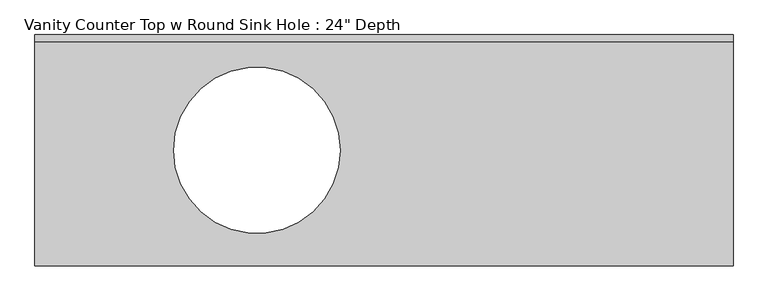
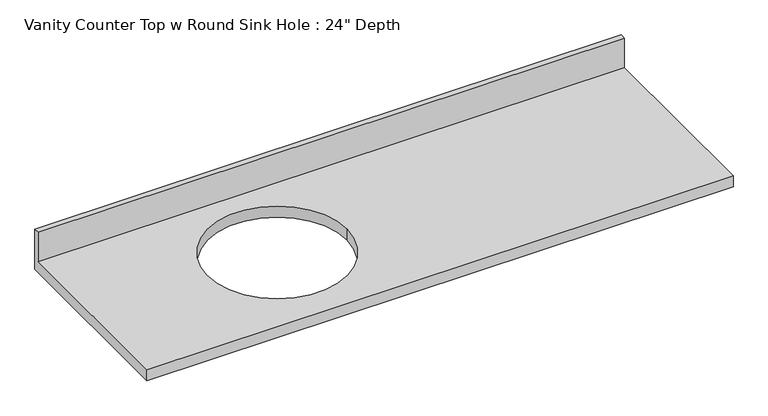
"""IFC4 building model written with IfcOpenShell, lengths in millimetres: furniture geometry."""

from ifc_helpers import new_model, si_unit, frame, origin, place, context, project, spatial, polyline, circle_curve, source, transform, mapped, element, save
from ifc_brep_helpers import plane_surface, revolved_surface, advanced_brep


def furniture_8bca8839(model_context):
    return source(origin(), model_context, "Body", "AdvancedBrep", [
        advanced_brep(
        [(-1327.4622951, -635.0, 787.4), (590.2377049, -635.0, 787.4), (590.2377049, -19.05, 787.4), (-1327.4622951, -19.05, 787.4), (-489.2622951, -317.5, 787.4), (-946.4622951, -317.5, 787.4), (590.2377049, 0.0, 749.3), (590.2377049, -635.0, 749.3), (-1327.4622951, -635.0, 749.3), (-1327.4622951, 0.0, 749.3), (-946.4622951, -317.5, 749.3), (-489.2622951, -317.5, 749.3), (-1327.4622951, 0.0, 889.0), (590.2377049, 0.0, 889.0), (-1327.4622951, -19.05, 889.0), (590.2377049, -19.05, 889.0)],
        [
            (0, 1),
            (1, 2),
            (2, 3),
            (3, 0),
            (4, 5, circle_curve(frame((-717.8622951, -317.5, 787.4), z_axis=(0.0, 0.0, -1.0), x_axis=(1.0, 0.0, 0.0)), 228.6)),
            (5, 4, circle_curve(frame((-717.8622951, -317.5, 787.4), z_axis=(0.0, 0.0, -1.0), x_axis=(1.0, 0.0, 0.0)), 228.6)),
            (6, 7),
            (7, 8),
            (8, 9),
            (9, 6),
            (10, 11, circle_curve(frame((-717.8622951, -317.5, 749.3), z_axis=(0.0, 0.0, 1.0), x_axis=(1.0, 0.0, 0.0)), 228.6)),
            (11, 10, circle_curve(frame((-717.8622951, -317.5, 749.3), z_axis=(0.0, 0.0, 1.0), x_axis=(1.0, 0.0, 0.0)), 228.6)),
            (9, 12),
            (12, 13),
            (13, 6),
            (8, 0),
            (3, 14),
            (14, 12),
            (7, 1),
            (13, 15),
            (15, 2),
            (14, 15),
            (4, 11),
            (10, 5),
        ],
        [
            plane_surface(frame((-1327.4622951, 0.0, 787.4), z_axis=(0.0, 0.0, 1.0), x_axis=(-1.0, 0.0, 0.0))),
            plane_surface(frame((-1327.4622951, 0.0, 749.3), z_axis=(0.0, 0.0, -1.0), x_axis=(1.0, 0.0, 0.0))),
            plane_surface(frame((590.2377049, 0.0, 787.4), z_axis=(0.0, 1.0, 0.0), x_axis=(0.0, 0.0, -1.0))),
            plane_surface(frame((-1327.4622951, 0.0, 787.4), z_axis=(-1.0, 0.0, 0.0), x_axis=(0.0, 0.0, -1.0))),
            plane_surface(frame((-1327.4622951, -635.0, 787.4), z_axis=(0.0, -1.0, 0.0), x_axis=(0.0, 0.0, -1.0))),
            plane_surface(frame((590.2377049, -635.0, 787.4), z_axis=(1.0, 0.0, 0.0), x_axis=(0.0, 0.0, -1.0))),
            plane_surface(frame((-1327.4622951, 0.0, 889.0), z_axis=(0.0, 0.0, 1.0), x_axis=(0.0, -1.0, 0.0))),
            plane_surface(frame((-1327.4622951, -19.05, 889.0), z_axis=(0.0, -1.0, 0.0), x_axis=(0.0, 0.0, -1.0))),
            revolved_surface(polyline([(-489.26229509999996, -317.5, 787.4), (-489.26229509999996, -317.5, 749.3)]), (-717.8622951, -317.5, 749.3), (0.0, 0.0, 1.0)),
        ],
        [
            (0, [[1, 2, 3, 4], [5, 6]]),
            (1, [[7, 8, 9, 10], [11, 12]]),
            (2, [[-10, 13, 14, 15]]),
            (3, [[-9, 16, -4, 17, 18, -13]]),
            (4, [[-1, -16, -8, 19]]),
            (5, [[-7, -15, 20, 21, -2, -19]]),
            (6, [[-18, 22, -20, -14]]),
            (7, [[-22, -17, -3, -21]]),
            (8, [[23, -11, 24, -5]]),
            (8, [[-23, -6, -24, -12]]),
        ],
    ),
    ])


if __name__ == "__main__":
    model = new_model("IFC4")
    model_context = context("Model", 3, world=origin())
    ifc_project = project(units=[si_unit("LENGTHUNIT", "METRE", prefix="MILLI")], contexts=[model_context])
    site = spatial("IfcSite", under=ifc_project)
    building = spatial("IfcBuilding", under=site)
    placement = place(None, origin())
    furniture_shape = furniture_8bca8839(model_context)
    element("IfcFurniture", 1, ObjectType="Vanity Counter Top w Round Sink Hole : 24\" Depth", at=placement, inside=building, context=model_context, shape_type="MappedRepresentation", body=[
        mapped(furniture_shape, transform((0.0, 0.0, 0.0), x_axis=(1.0, 0.0, 0.0), y_axis=(0.0, 1.0, 0.0), z_axis=(0.0, 0.0, 1.0))),
    ])
    save(model, "model.ifc")

# Revit data of these elements
# Type "Vanity Counter Top w Round Sink Hole : 24\" Depth"
#   Assembly Code = "C1030400"
#   Counter Thickness = 0' - 1 1/2"
#   Depth = 2' - 1"
#   Height = 2' - 7"
#   Length [instance default] = 4' - 0"
#   Sink Location [instance default] = 2' - 0"
#   Sink Location To Wall [instance default] = 0' - 4"
#   Sink Opening Width [instance default] = 1' - 5"
#   Counter Top Material = Laminate, Blue, Matte
#   Default Elevation = 0
# Element 1 (IfcFurniture, "Vanity Counter Top w Round Sink Hole : 24\" Depth")
#   Length = 6' - 3 1/2"
#   Materials on its faces: "Laminate, Blue, Matte"
# Materials
#   "Laminate, Blue, Matte": class "Plastic", colour RGB 85 101 155, transparency 0, Description = "Plastic Laminate - Blue, Matte", Cost = 0
